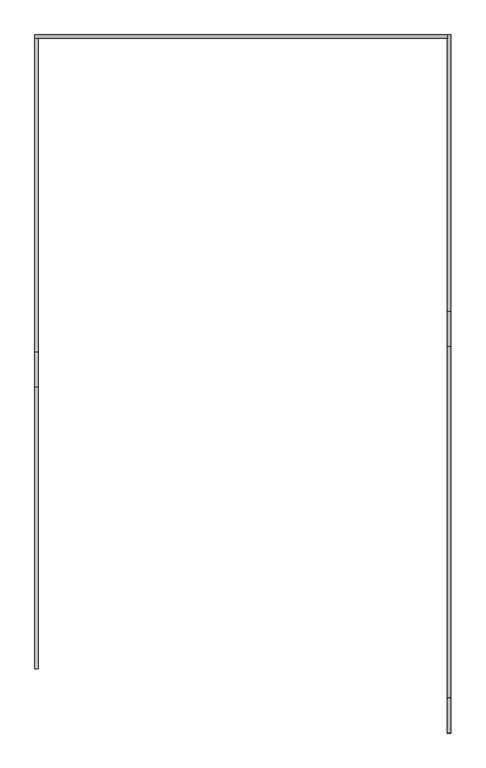
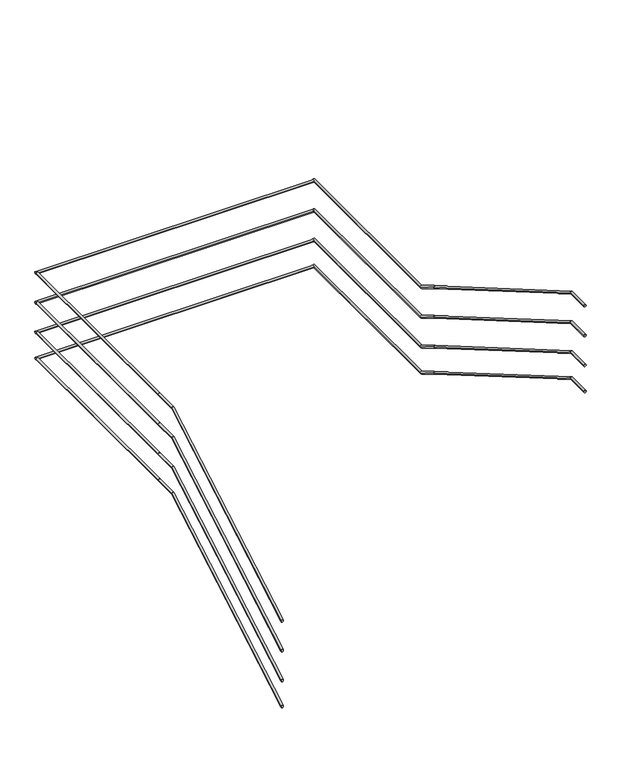
"""IFC4 building model written with IfcOpenShell, lengths in millimetres: railing geometry."""

import ifcopenshell
import ifcopenshell.guid

model = None  # the IFC model being written
_history = None  # IfcOwnerHistory: only IFC2X3 demands one
_inside = {}  # id of a spatial element -> (the spatial element, [elements in it])
_under = {}  # id of a project, library or spatial element -> (it, [spatial elements below it])
_declared = {}  # id of a project -> (the project, [libraries it declares])
_typed = {}  # id of a type object -> (the type object, [elements of that type])
_made_of = {}  # id of a material, layer set ... -> (it, [elements and type objects made of it])


def new_model(schema):
    """Start an empty IFC model of exactly this schema.

    Asked for "IFC4X3", IfcOpenShell would pick the latest addendum, in which some entities
    have other attributes; the version numbers below select the first issue.
    IFC2X3 requires an IfcOwnerHistory on every rooted entity: one is made here for all.
    """
    global model, _history
    if schema == "IFC4X3":
        model = ifcopenshell.file(schema_version=(4, 3, 0, 0))
    else:
        model = ifcopenshell.file(schema=schema)
    _inside.clear()
    _under.clear()
    _declared.clear()
    _typed.clear()
    _made_of.clear()
    _history = None
    if model.schema == "IFC2X3":
        org = make("IfcOrganization", Name="unknown")
        user = make(
            "IfcPersonAndOrganization",
            ThePerson=make("IfcPerson", FamilyName="unknown"),
            TheOrganization=org,
        )
        app = make(
            "IfcApplication",
            ApplicationDeveloper=org,
            Version="unknown",
            ApplicationFullName="unknown",
            ApplicationIdentifier="unknown",
        )
        _history = make(
            "IfcOwnerHistory",
            OwningUser=user,
            OwningApplication=app,
            ChangeAction="ADDED",
            CreationDate=0,
        )
    return model


def make(cls, **values):
    """One entity of the class cls with the attributes given. An attribute that is None is left unset."""
    return model.create_entity(
        cls, **{name: value for name, value in values.items() if value is not None}
    )


def rooted(cls, **values):
    """An entity with a GlobalId (a new one), such as an element, a storey or a relation."""
    return make(cls, GlobalId=ifcopenshell.guid.new(), OwnerHistory=_history, **values)


def si_unit(unit_type, name, prefix=None):
    """IfcSIUnit, for example si_unit("LENGTHUNIT", "METRE", prefix="MILLI")."""
    return make("IfcSIUnit", UnitType=unit_type, Prefix=prefix, Name=name)


def assignment(units):
    """IfcUnitAssignment: the units of a project."""
    return None if units is None else make("IfcUnitAssignment", Units=units)


def point(xyz):
    """IfcCartesianPoint."""
    return None if xyz is None else make("IfcCartesianPoint", Coordinates=xyz)


def direction(xyz):
    """IfcDirection."""
    return None if xyz is None else make("IfcDirection", DirectionRatios=xyz)


def frame(location, z_axis=None, x_axis=None):
    """IfcAxis2Placement3D, a coordinate frame: its origin and axes. An axis left out is left unset."""
    return make(
        "IfcAxis2Placement3D",
        Location=point(location),
        Axis=direction(z_axis),
        RefDirection=direction(x_axis),
    )


def origin():
    """The frame at (0, 0, 0) with its axes left unset."""
    return frame((0.0, 0.0, 0.0))


def place(relative_to, where):
    """IfcLocalPlacement: puts the frame where relative to a parent placement (None: the world)."""
    return make(
        "IfcLocalPlacement", PlacementRelTo=relative_to, RelativePlacement=where
    )


def context(
    kind, dimensions, precision=None, world=None, true_north=None, identifier=None
):
    """IfcGeometricRepresentationContext, for example the 3D "Model" context."""
    return make(
        "IfcGeometricRepresentationContext",
        ContextIdentifier=identifier,
        ContextType=kind,
        CoordinateSpaceDimension=dimensions,
        Precision=precision,
        WorldCoordinateSystem=world,
        TrueNorth=true_north,
    )


def project(units=None, contexts=None):
    """IfcProject with its units and contexts."""
    return rooted(
        "IfcProject",
        Name="project",
        RepresentationContexts=contexts,
        UnitsInContext=assignment(units),
    )


def spatial(cls, under=None, at=None, **own):
    """A site, building, storey or space (cls), placed at a placement, below another one or the project."""
    s = rooted(cls, ObjectPlacement=at, **own)
    if under is not None:
        _under.setdefault(under.id(), (under, []))[1].append(s)
    return s


def circle_curve(where, radius):
    """IfcCircle in the frame where."""
    return make("IfcCircle", Position=where, Radius=radius)


def ellipse_curve(where, semi_axis1, semi_axis2):
    """IfcEllipse in the frame where."""
    return make(
        "IfcEllipse", Position=where, SemiAxis1=semi_axis1, SemiAxis2=semi_axis2
    )


def shape(context_of_items, identifier, shape_type, items):
    """IfcShapeRepresentation: the items that make up one representation, for example the "Body"."""
    return make(
        "IfcShapeRepresentation",
        ContextOfItems=context_of_items,
        RepresentationIdentifier=identifier,
        RepresentationType=shape_type,
        Items=items,
    )


def source(mapping_origin, context_of_items, identifier, shape_type, items):
    """IfcRepresentationMap: a shape defined once, which mapped items show again and again."""
    return make(
        "IfcRepresentationMap",
        MappingOrigin=mapping_origin,
        MappedRepresentation=shape(context_of_items, identifier, shape_type, items),
    )


def transform(
    local_origin,
    x_axis=None,
    y_axis=None,
    z_axis=None,
    scale=None,
    scale2=None,
    scale3=None,
    uniform=True,
):
    """IfcCartesianTransformationOperator3D, or its non-uniform kind. x_axis, y_axis, z_axis: its Axis1, 2, 3."""
    if uniform:
        return make(
            "IfcCartesianTransformationOperator3D",
            Axis1=direction(x_axis),
            Axis2=direction(y_axis),
            LocalOrigin=point(local_origin),
            Scale=scale,
            Axis3=direction(z_axis),
        )
    return make(
        "IfcCartesianTransformationOperator3DnonUniform",
        Axis1=direction(x_axis),
        Axis2=direction(y_axis),
        LocalOrigin=point(local_origin),
        Scale=scale,
        Axis3=direction(z_axis),
        Scale2=scale2,
        Scale3=scale3,
    )


def mapped(mapping_source, mapping_target):
    """IfcMappedItem: shows the shape of a source again, moved by a transform."""
    return make(
        "IfcMappedItem", MappingSource=mapping_source, MappingTarget=mapping_target
    )


def made_of(thing, what):
    """Note that an element or type object is made of a material, layer set ...; save() writes the relation."""
    if what is not None:
        _made_of.setdefault(what.id(), (what, []))[1].append(thing)
    return thing


def element(
    cls,
    number,
    at=None,
    inside=None,
    cuts=None,
    type_object=None,
    material=None,
    context=None,
    identifier="Body",
    shape_type=None,
    held_by="IfcProductDefinitionShape",
    body=None,
    shapes=None,
    **own,
):
    """One element of the class cls, such as IfcWall. Its Tag is "e" and its number.

    at: its placement. inside: the storey or other place that contains it. cuts: it is an
    opening in that element (IfcRelVoidsElement). A single representation is given by context,
    identifier, shape_type and body (its items); several are given by shapes. held_by: the class
    of the entity that holds the representations. save() writes the other relations.
    """
    e = rooted(cls, Tag="e%d" % number, ObjectPlacement=at, **own)
    if body is not None:
        shapes = [shape(context, identifier, shape_type, body)]
    if shapes is not None:
        e.Representation = make(held_by, Representations=shapes)
    if inside is not None:
        _inside.setdefault(inside.id(), (inside, []))[1].append(e)
    if cuts is not None:
        rooted(
            "IfcRelVoidsElement", RelatingBuildingElement=cuts, RelatedOpeningElement=e
        )
    if type_object is not None:
        _typed.setdefault(type_object.id(), (type_object, []))[1].append(e)
    return made_of(e, material)


def aggregate(whole, parts):
    """IfcRelAggregates: a whole, such as a stair, and the parts it consists of."""
    return rooted("IfcRelAggregates", RelatingObject=whole, RelatedObjects=parts)


def save(model, path):
    """Write the relations noted so far, then the file.

    IfcRelAggregates (storeys below a building ...), IfcRelContainedInSpatialStructure (elements
    in a storey), IfcRelDefinesByType, IfcRelAssociatesMaterial and IfcRelDeclares: one each for
    every whole, place, type object, material and project.
    """
    for whole, parts in _under.values():
        aggregate(whole, parts)
    for where, things in _inside.values():
        rooted(
            "IfcRelContainedInSpatialStructure",
            RelatedElements=things,
            RelatingStructure=where,
        )
    for kind, things in _typed.values():
        rooted("IfcRelDefinesByType", RelatedObjects=things, RelatingType=kind)
    for what, things in _made_of.values():
        rooted("IfcRelAssociatesMaterial", RelatedObjects=things, RelatingMaterial=what)
    for by, libraries in _declared.values():
        rooted("IfcRelDeclares", RelatingContext=by, RelatedDefinitions=libraries)
    model.write(path)


def plane_surface(at):
    """IfcPlane: the flat surface through the origin of the frame at, square to its z axis."""
    return make("IfcPlane", Position=at)


def cylinder_surface(at, radius):
    """IfcCylindricalSurface: all points at the distance radius from the z axis of the frame at."""
    return make("IfcCylindricalSurface", Position=at, Radius=radius)


def advanced_brep(points, edges, surfaces, faces):
    """IfcAdvancedBrep: a solid bounded by faces that lie on surfaces and meet in shared edges.

    An edge is (start, end): straight between two places in points (the first is 0);
    or (start, end, curve); or (start, end, curve, False) where it runs against its curve.
    A face is (place in surfaces, loops), or (place, loops, False) where it looks against
    its surface's normal. A loop lists edges by number (the first is 1), with a minus sign
    where the edge is run from its end to its start. The first loop is the outer one.
    """
    corners = [point(p) for p in points]
    vertices = [make("IfcVertexPoint", VertexGeometry=c) for c in corners]
    made = []
    for start, end, *more in edges:
        made.append(
            make(
                "IfcEdgeCurve",
                EdgeStart=vertices[start],
                EdgeEnd=vertices[end],
                EdgeGeometry=more[0] if more else make("IfcPolyline", Points=[corners[start], corners[end]]),
                SameSense=more[1] if len(more) > 1 else True,
            )
        )
    hull = []
    for where, loops, *sense in faces:
        bounds = []
        for j, loop in enumerate(loops):
            ring = [make("IfcOrientedEdge", EdgeElement=made[abs(k) - 1], Orientation=k > 0) for k in loop]
            bounds.append(
                make(
                    "IfcFaceOuterBound" if j == 0 else "IfcFaceBound",
                    Bound=make("IfcEdgeLoop", EdgeList=ring),
                    Orientation=True,
                )
            )
        hull.append(make("IfcAdvancedFace", Bounds=bounds, FaceSurface=surfaces[where], SameSense=sense[0] if sense else True))
    return make("IfcAdvancedBrep", Outer=make("IfcClosedShell", CfsFaces=hull))


def railing_c3b53c4a(model_context):
    return source(origin(), model_context, "Body", "AdvancedBrep", [
        advanced_brep(
        [(51115.4, 12129.5208589, 7307.5963084), (51085.4, 12129.5208589, 7307.5963084), (51115.4, 14533.576096, 8709.9618634), (51085.4, 14533.576096, 8709.9618634), (51115.4, 14829.5208589, 8709.9618634), (51085.4, 14829.5208589, 8709.9618634)],
        [
            (0, 1, ellipse_curve(frame((51100.4, 12129.5208589, 7307.5963084), z_axis=(0.0, -1.0, 0.0), x_axis=(0.0, 0.0, -1.0)), 17.365555, 15.0)),
            (1, 0, ellipse_curve(frame((51100.4, 12129.5208589, 7307.5963084), z_axis=(0.0, -1.0, 0.0), x_axis=(0.0, 0.0, -1.0)), 17.365555, 15.0)),
            (0, 2),
            (2, 3, ellipse_curve(frame((51100.4, 14533.576096, 8709.9618634), z_axis=(0.0, -0.9653442134540491, -0.26097997921446625), x_axis=(0.0, 0.2609799792144657, -0.9653442134540494)), 15.5384989, 15.0)),
            (3, 1),
            (3, 2, ellipse_curve(frame((51100.4, 14533.576096, 8709.9618634), z_axis=(0.0, -0.9653442134540491, -0.26097997921446625), x_axis=(0.0, 0.2609799792144657, -0.9653442134540494)), 15.5384989, 15.0)),
            (4, 5, circle_curve(frame((51100.4, 14829.5208589, 8709.9618634), z_axis=(0.0, 1.0, 0.0), x_axis=(-1.0, 0.0, 0.0)), 15.0)),
            (5, 4, circle_curve(frame((51100.4, 14829.5208589, 8709.9618634), z_axis=(0.0, 1.0, 0.0), x_axis=(-1.0, 0.0, 0.0)), 15.0)),
            (2, 4),
            (5, 3),
        ],
        [
            plane_surface(frame((51100.4, 12129.5208589, 7324.9618634), z_axis=(0.0, -1.0, 0.0), x_axis=(0.0, 0.0, 1.0))),
            cylinder_surface(frame((51100.4, 12137.0789243, 7312.0051799), z_axis=(0.0, -0.8637789008984336, -0.5038710255240861), x_axis=(-1.0, 0.0, 0.0)), 15.0),
            plane_surface(frame((51100.4, 14829.5208589, 8724.9618634), z_axis=(0.0, 1.0, 0.0), x_axis=(0.0, 0.0, 1.0))),
            cylinder_surface(frame((51100.4, 14529.5208589, 8709.9618634), z_axis=(0.0, -1.0, 0.0), x_axis=(-1.0, 0.0, 0.0)), 15.0),
        ],
        [
            (0, [[1, 2]]),
            (1, [[-1, 3, 4, 5]]),
            (1, [[-2, -5, 6, -3]]),
            (2, [[7, 8]]),
            (3, [[-4, 9, -8, 10]]),
            (3, [[-6, -10, -7, -9]]),
        ],
    ),
        advanced_brep(
        [(51115.4, 14829.5208589, 8709.9618634), (51085.4, 14829.5208589, 8709.9618634), (51115.4, 17509.1208589, 8709.9618634), (51085.4, 17509.1208589, 8709.9618634)],
        [
            (0, 1, circle_curve(frame((51100.4, 14829.5208589, 8709.9618634), z_axis=(0.0, -1.0, 0.0), x_axis=(-1.0, 0.0, 0.0)), 15.0)),
            (1, 0, circle_curve(frame((51100.4, 14829.5208589, 8709.9618634), z_axis=(0.0, -1.0, 0.0), x_axis=(-1.0, 0.0, 0.0)), 15.0)),
            (2, 3, circle_curve(frame((51100.4, 17509.1208589, 8709.9618634), z_axis=(0.0, 1.0, 0.0), x_axis=(-1.0, 0.0, 0.0)), 15.0)),
            (3, 2, circle_curve(frame((51100.4, 17509.1208589, 8709.9618634), z_axis=(0.0, 1.0, 0.0), x_axis=(-1.0, 0.0, 0.0)), 15.0)),
            (0, 2),
            (3, 1),
        ],
        [
            plane_surface(frame((51100.4, 14829.5208589, 8724.9618634), z_axis=(0.0, -1.0, 0.0), x_axis=(0.0, 0.0, 1.0))),
            plane_surface(frame((51100.4, 17509.1208589, 8724.9618634), z_axis=(0.0, 1.0, 0.0), x_axis=(0.0, 0.0, 1.0))),
            cylinder_surface(frame((51100.4, 14829.5208589, 8709.9618634), z_axis=(0.0, -1.0, 0.0), x_axis=(-1.0, 0.0, 0.0)), 15.0),
        ],
        [
            (0, [[1, 2]]),
            (1, [[3, 4]]),
            (2, [[-1, 5, -4, 6]]),
            (2, [[-2, -6, -3, -5]]),
        ],
    ),
        advanced_brep(
        [(51085.4, 17509.1208589, 8709.9618634), (51085.4, 17539.1208589, 8709.9618634), (54609.6, 17509.1208589, 8709.9618634), (54609.6, 17539.1208589, 8709.9618634)],
        [
            (0, 1, circle_curve(frame((51085.4, 17524.1208589, 8709.9618634), z_axis=(-1.0, 0.0, 0.0), x_axis=(0.0, 1.0, 0.0)), 15.0)),
            (1, 0, circle_curve(frame((51085.4, 17524.1208589, 8709.9618634), z_axis=(-1.0, 0.0, 0.0), x_axis=(0.0, 1.0, 0.0)), 15.0)),
            (2, 3, circle_curve(frame((54609.6, 17524.1208589, 8709.9618634), z_axis=(1.0, 0.0, 0.0), x_axis=(0.0, 1.0, 0.0)), 15.0)),
            (3, 2, circle_curve(frame((54609.6, 17524.1208589, 8709.9618634), z_axis=(1.0, 0.0, 0.0), x_axis=(0.0, 1.0, 0.0)), 15.0)),
            (0, 2),
            (3, 1),
        ],
        [
            plane_surface(frame((51085.4, 17524.1208589, 8724.9618634), z_axis=(-1.0, 0.0, 0.0), x_axis=(0.0, 1.0, 0.0))),
            plane_surface(frame((54609.6, 17524.1208589, 8724.9618634), z_axis=(1.0, 0.0, 0.0), x_axis=(0.0, 1.0, 0.0))),
            cylinder_surface(frame((51085.4, 17524.1208589, 8709.9618634), z_axis=(-1.0, 0.0, 0.0), x_axis=(0.0, 1.0, 0.0)), 15.0),
        ],
        [
            (0, [[1, 2]]),
            (1, [[3, 4]]),
            (2, [[-1, 5, -4, 6]]),
            (2, [[-2, -6, -3, -5]]),
        ],
    ),
        advanced_brep(
        [(54609.6, 17539.1208589, 8709.9618634), (54639.6, 17539.1208589, 8709.9618634), (54609.6, 15175.4656218, 8709.9618634), (54639.6, 15175.4656218, 8709.9618634), (54609.6, 14879.5208589, 8882.5963084), (54639.6, 14879.5208589, 8882.5963084)],
        [
            (0, 1, circle_curve(frame((54624.6, 17539.1208589, 8709.9618634), z_axis=(0.0, 1.0, 0.0), x_axis=(1.0, 0.0, 0.0)), 15.0)),
            (1, 0, circle_curve(frame((54624.6, 17539.1208589, 8709.9618634), z_axis=(0.0, 1.0, 0.0), x_axis=(1.0, 0.0, 0.0)), 15.0)),
            (0, 2),
            (2, 3, ellipse_curve(frame((54624.6, 15175.4656218, 8709.9618634), z_axis=(0.0, 0.9653442134540493, -0.26097997921446586), x_axis=(0.0, 0.2609799792144653, 0.9653442134540493)), 15.5384989, 15.0)),
            (3, 1),
            (3, 2, ellipse_curve(frame((54624.6, 15175.4656218, 8709.9618634), z_axis=(0.0, 0.9653442134540493, -0.26097997921446586), x_axis=(0.0, 0.2609799792144653, 0.9653442134540493)), 15.5384989, 15.0)),
            (4, 5, ellipse_curve(frame((54624.6, 14879.5208589, 8882.5963084), z_axis=(0.0, -1.0, 0.0), x_axis=(0.0, 0.0, -1.0)), 17.365555, 15.0)),
            (5, 4, ellipse_curve(frame((54624.6, 14879.5208589, 8882.5963084), z_axis=(0.0, -1.0, 0.0), x_axis=(0.0, 0.0, -1.0)), 17.365555, 15.0)),
            (2, 4),
            (5, 3),
        ],
        [
            plane_surface(frame((54624.6, 17539.1208589, 8724.9618634), z_axis=(0.0, 1.0, 0.0), x_axis=(0.0, 0.0, -1.0))),
            cylinder_surface(frame((54624.6, 17539.1208589, 8709.9618634), z_axis=(0.0, 1.0, 0.0), x_axis=(1.0, 0.0, 0.0)), 15.0),
            plane_surface(frame((54624.6, 14879.5208589, 8899.9618634), z_axis=(0.0, -1.0, 0.0), x_axis=(0.0, 0.0, -1.0))),
            cylinder_surface(frame((54624.6, 15171.9627935, 8712.0051799), z_axis=(0.0, 0.8637789008984339, -0.5038710255240854), x_axis=(1.0, 0.0, 0.0)), 15.0),
        ],
        [
            (0, [[1, 2]]),
            (1, [[-1, 3, 4, 5]]),
            (1, [[-2, -5, 6, -3]]),
            (2, [[7, 8]]),
            (3, [[-4, 9, -8, 10]]),
            (3, [[-6, -10, -7, -9]]),
        ],
    ),
        advanced_brep(
        [(54609.6, 14879.5208589, 8882.5963084), (54639.6, 14879.5208589, 8882.5963084), (54609.6, 11875.4656218, 10634.9618634), (54639.6, 11875.4656218, 10634.9618634), (54609.6, 11579.5208589, 10634.9618634), (54639.6, 11579.5208589, 10634.9618634)],
        [
            (0, 1, ellipse_curve(frame((54624.6, 14879.5208589, 8882.5963084), z_axis=(0.0, 1.0, 0.0), x_axis=(0.0, 0.0, -1.0)), 17.365555, 15.0)),
            (1, 0, ellipse_curve(frame((54624.6, 14879.5208589, 8882.5963084), z_axis=(0.0, 1.0, 0.0), x_axis=(0.0, 0.0, -1.0)), 17.365555, 15.0)),
            (0, 2),
            (2, 3, ellipse_curve(frame((54624.6, 11875.4656218, 10634.9618634), z_axis=(0.0, 0.9653442134540491, -0.26097997921446625), x_axis=(0.0, -0.2609799792144661, -0.9653442134540492)), 15.5384989, 15.0)),
            (3, 1),
            (3, 2, ellipse_curve(frame((54624.6, 11875.4656218, 10634.9618634), z_axis=(0.0, 0.9653442134540491, -0.26097997921446625), x_axis=(0.0, -0.2609799792144661, -0.9653442134540492)), 15.5384989, 15.0)),
            (4, 5, circle_curve(frame((54624.6, 11579.5208589, 10634.9618634), z_axis=(0.0, -1.0, 0.0), x_axis=(1.0, 0.0, 0.0)), 15.0)),
            (5, 4, circle_curve(frame((54624.6, 11579.5208589, 10634.9618634), z_axis=(0.0, -1.0, 0.0), x_axis=(1.0, 0.0, 0.0)), 15.0)),
            (2, 4),
            (5, 3),
        ],
        [
            plane_surface(frame((54624.6, 14879.5208589, 8899.9618634), z_axis=(0.0, 1.0, 0.0), x_axis=(0.0, 0.0, -1.0))),
            cylinder_surface(frame((54624.6, 14871.9627935, 8887.0051799), z_axis=(0.0, 0.8637789008984335, -0.5038710255240861), x_axis=(1.0, 0.0, 0.0)), 15.0),
            plane_surface(frame((54624.6, 11579.5208589, 10649.9618634), z_axis=(0.0, -1.0, 0.0), x_axis=(0.0, 0.0, -1.0))),
            cylinder_surface(frame((54624.6, 11879.5208589, 10634.9618634), z_axis=(0.0, 1.0, 0.0), x_axis=(1.0, 0.0, 0.0)), 15.0),
        ],
        [
            (0, [[1, 2]]),
            (1, [[-1, 3, 4, 5]]),
            (1, [[-2, -5, 6, -3]]),
            (2, [[7, 8]]),
            (3, [[-4, 9, -8, 10]]),
            (3, [[-6, -10, -7, -9]]),
        ],
    ),
        advanced_brep(
        [(51115.4, 12129.5208589, 6507.5963084), (51085.4, 12129.5208589, 6507.5963084), (51115.4, 14533.576096, 7909.9618634), (51085.4, 14533.576096, 7909.9618634), (51115.4, 14829.5208589, 7909.9618634), (51085.4, 14829.5208589, 7909.9618634)],
        [
            (0, 1, ellipse_curve(frame((51100.4, 12129.5208589, 6507.5963084), z_axis=(0.0, -1.0, 0.0), x_axis=(0.0, 0.0, -1.0)), 17.365555, 15.0)),
            (1, 0, ellipse_curve(frame((51100.4, 12129.5208589, 6507.5963084), z_axis=(0.0, -1.0, 0.0), x_axis=(0.0, 0.0, -1.0)), 17.365555, 15.0)),
            (0, 2),
            (2, 3, ellipse_curve(frame((51100.4, 14533.576096, 7909.9618634), z_axis=(0.0, -0.9653442134540491, -0.26097997921446625), x_axis=(0.0, 0.2609799792144657, -0.9653442134540494)), 15.5384989, 15.0)),
            (3, 1),
            (3, 2, ellipse_curve(frame((51100.4, 14533.576096, 7909.9618634), z_axis=(0.0, -0.9653442134540491, -0.26097997921446625), x_axis=(0.0, 0.2609799792144657, -0.9653442134540494)), 15.5384989, 15.0)),
            (4, 5, circle_curve(frame((51100.4, 14829.5208589, 7909.9618634), z_axis=(0.0, 1.0, 0.0), x_axis=(-1.0, 0.0, 0.0)), 15.0)),
            (5, 4, circle_curve(frame((51100.4, 14829.5208589, 7909.9618634), z_axis=(0.0, 1.0, 0.0), x_axis=(-1.0, 0.0, 0.0)), 15.0)),
            (2, 4),
            (5, 3),
        ],
        [
            plane_surface(frame((51100.4, 12129.5208589, 6524.9618634), z_axis=(0.0, -1.0, 0.0), x_axis=(0.0, 0.0, 1.0))),
            cylinder_surface(frame((51100.4, 12137.0789243, 6512.0051799), z_axis=(0.0, -0.8637789008984336, -0.5038710255240861), x_axis=(-1.0, 0.0, 0.0)), 15.0),
            plane_surface(frame((51100.4, 14829.5208589, 7924.9618634), z_axis=(0.0, 1.0, 0.0), x_axis=(0.0, 0.0, 1.0))),
            cylinder_surface(frame((51100.4, 14529.5208589, 7909.9618634), z_axis=(0.0, -1.0, 0.0), x_axis=(-1.0, 0.0, 0.0)), 15.0),
        ],
        [
            (0, [[1, 2]]),
            (1, [[-1, 3, 4, 5]]),
            (1, [[-2, -5, 6, -3]]),
            (2, [[7, 8]]),
            (3, [[-4, 9, -8, 10]]),
            (3, [[-6, -10, -7, -9]]),
        ],
    ),
        advanced_brep(
        [(51115.4, 14829.5208589, 7909.9618634), (51085.4, 14829.5208589, 7909.9618634), (51115.4, 17509.1208589, 7909.9618634), (51085.4, 17509.1208589, 7909.9618634)],
        [
            (0, 1, circle_curve(frame((51100.4, 14829.5208589, 7909.9618634), z_axis=(0.0, -1.0, 0.0), x_axis=(-1.0, 0.0, 0.0)), 15.0)),
            (1, 0, circle_curve(frame((51100.4, 14829.5208589, 7909.9618634), z_axis=(0.0, -1.0, 0.0), x_axis=(-1.0, 0.0, 0.0)), 15.0)),
            (2, 3, circle_curve(frame((51100.4, 17509.1208589, 7909.9618634), z_axis=(0.0, 1.0, 0.0), x_axis=(-1.0, 0.0, 0.0)), 15.0)),
            (3, 2, circle_curve(frame((51100.4, 17509.1208589, 7909.9618634), z_axis=(0.0, 1.0, 0.0), x_axis=(-1.0, 0.0, 0.0)), 15.0)),
            (0, 2),
            (3, 1),
        ],
        [
            plane_surface(frame((51100.4, 14829.5208589, 7924.9618634), z_axis=(0.0, -1.0, 0.0), x_axis=(0.0, 0.0, 1.0))),
            plane_surface(frame((51100.4, 17509.1208589, 7924.9618634), z_axis=(0.0, 1.0, 0.0), x_axis=(0.0, 0.0, 1.0))),
            cylinder_surface(frame((51100.4, 14829.5208589, 7909.9618634), z_axis=(0.0, -1.0, 0.0), x_axis=(-1.0, 0.0, 0.0)), 15.0),
        ],
        [
            (0, [[1, 2]]),
            (1, [[3, 4]]),
            (2, [[-1, 5, -4, 6]]),
            (2, [[-2, -6, -3, -5]]),
        ],
    ),
        advanced_brep(
        [(51085.4, 17509.1208589, 7909.9618634), (51085.4, 17539.1208589, 7909.9618634), (54609.6, 17509.1208589, 7909.9618634), (54609.6, 17539.1208589, 7909.9618634)],
        [
            (0, 1, circle_curve(frame((51085.4, 17524.1208589, 7909.9618634), z_axis=(-1.0, 0.0, 0.0), x_axis=(0.0, 1.0, 0.0)), 15.0)),
            (1, 0, circle_curve(frame((51085.4, 17524.1208589, 7909.9618634), z_axis=(-1.0, 0.0, 0.0), x_axis=(0.0, 1.0, 0.0)), 15.0)),
            (2, 3, circle_curve(frame((54609.6, 17524.1208589, 7909.9618634), z_axis=(1.0, 0.0, 0.0), x_axis=(0.0, 1.0, 0.0)), 15.0)),
            (3, 2, circle_curve(frame((54609.6, 17524.1208589, 7909.9618634), z_axis=(1.0, 0.0, 0.0), x_axis=(0.0, 1.0, 0.0)), 15.0)),
            (0, 2),
            (3, 1),
        ],
        [
            plane_surface(frame((51085.4, 17524.1208589, 7924.9618634), z_axis=(-1.0, 0.0, 0.0), x_axis=(0.0, 1.0, 0.0))),
            plane_surface(frame((54609.6, 17524.1208589, 7924.9618634), z_axis=(1.0, 0.0, 0.0), x_axis=(0.0, 1.0, 0.0))),
            cylinder_surface(frame((51085.4, 17524.1208589, 7909.9618634), z_axis=(-1.0, 0.0, 0.0), x_axis=(0.0, 1.0, 0.0)), 15.0),
        ],
        [
            (0, [[1, 2]]),
            (1, [[3, 4]]),
            (2, [[-1, 5, -4, 6]]),
            (2, [[-2, -6, -3, -5]]),
        ],
    ),
        advanced_brep(
        [(54609.6, 17539.1208589, 7909.9618634), (54639.6, 17539.1208589, 7909.9618634), (54609.6, 15175.4656218, 7909.9618634), (54639.6, 15175.4656218, 7909.9618634), (54609.6, 14879.5208589, 8082.5963084), (54639.6, 14879.5208589, 8082.5963084)],
        [
            (0, 1, circle_curve(frame((54624.6, 17539.1208589, 7909.9618634), z_axis=(0.0, 1.0, 0.0), x_axis=(1.0, 0.0, 0.0)), 15.0)),
            (1, 0, circle_curve(frame((54624.6, 17539.1208589, 7909.9618634), z_axis=(0.0, 1.0, 0.0), x_axis=(1.0, 0.0, 0.0)), 15.0)),
            (0, 2),
            (2, 3, ellipse_curve(frame((54624.6, 15175.4656218, 7909.9618634), z_axis=(0.0, 0.9653442134540493, -0.26097997921446586), x_axis=(0.0, 0.2609799792144653, 0.9653442134540493)), 15.5384989, 15.0)),
            (3, 1),
            (3, 2, ellipse_curve(frame((54624.6, 15175.4656218, 7909.9618634), z_axis=(0.0, 0.9653442134540493, -0.26097997921446586), x_axis=(0.0, 0.2609799792144653, 0.9653442134540493)), 15.5384989, 15.0)),
            (4, 5, ellipse_curve(frame((54624.6, 14879.5208589, 8082.5963084), z_axis=(0.0, -1.0, 0.0), x_axis=(0.0, 0.0, -1.0)), 17.365555, 15.0)),
            (5, 4, ellipse_curve(frame((54624.6, 14879.5208589, 8082.5963084), z_axis=(0.0, -1.0, 0.0), x_axis=(0.0, 0.0, -1.0)), 17.365555, 15.0)),
            (2, 4),
            (5, 3),
        ],
        [
            plane_surface(frame((54624.6, 17539.1208589, 7924.9618634), z_axis=(0.0, 1.0, 0.0), x_axis=(0.0, 0.0, -1.0))),
            cylinder_surface(frame((54624.6, 17539.1208589, 7909.9618634), z_axis=(0.0, 1.0, 0.0), x_axis=(1.0, 0.0, 0.0)), 15.0),
            plane_surface(frame((54624.6, 14879.5208589, 8099.9618634), z_axis=(0.0, -1.0, 0.0), x_axis=(0.0, 0.0, -1.0))),
            cylinder_surface(frame((54624.6, 15171.9627935, 7912.0051799), z_axis=(0.0, 0.8637789008984339, -0.5038710255240854), x_axis=(1.0, 0.0, 0.0)), 15.0),
        ],
        [
            (0, [[1, 2]]),
            (1, [[-1, 3, 4, 5]]),
            (1, [[-2, -5, 6, -3]]),
            (2, [[7, 8]]),
            (3, [[-4, 9, -8, 10]]),
            (3, [[-6, -10, -7, -9]]),
        ],
    ),
        advanced_brep(
        [(54609.6, 14879.5208589, 8082.5963084), (54639.6, 14879.5208589, 8082.5963084), (54609.6, 11875.4656218, 9834.9618634), (54639.6, 11875.4656218, 9834.9618634), (54609.6, 11579.5208589, 9834.9618634), (54639.6, 11579.5208589, 9834.9618634)],
        [
            (0, 1, ellipse_curve(frame((54624.6, 14879.5208589, 8082.5963084), z_axis=(0.0, 1.0, 0.0), x_axis=(0.0, 0.0, -1.0)), 17.365555, 15.0)),
            (1, 0, ellipse_curve(frame((54624.6, 14879.5208589, 8082.5963084), z_axis=(0.0, 1.0, 0.0), x_axis=(0.0, 0.0, -1.0)), 17.365555, 15.0)),
            (0, 2),
            (2, 3, ellipse_curve(frame((54624.6, 11875.4656218, 9834.9618634), z_axis=(0.0, 0.9653442134540491, -0.26097997921446625), x_axis=(0.0, -0.2609799792144661, -0.9653442134540492)), 15.5384989, 15.0)),
            (3, 1),
            (3, 2, ellipse_curve(frame((54624.6, 11875.4656218, 9834.9618634), z_axis=(0.0, 0.9653442134540491, -0.26097997921446625), x_axis=(0.0, -0.2609799792144661, -0.9653442134540492)), 15.5384989, 15.0)),
            (4, 5, circle_curve(frame((54624.6, 11579.5208589, 9834.9618634), z_axis=(0.0, -1.0, 0.0), x_axis=(1.0, 0.0, 0.0)), 15.0)),
            (5, 4, circle_curve(frame((54624.6, 11579.5208589, 9834.9618634), z_axis=(0.0, -1.0, 0.0), x_axis=(1.0, 0.0, 0.0)), 15.0)),
            (2, 4),
            (5, 3),
        ],
        [
            plane_surface(frame((54624.6, 14879.5208589, 8099.9618634), z_axis=(0.0, 1.0, 0.0), x_axis=(0.0, 0.0, -1.0))),
            cylinder_surface(frame((54624.6, 14871.9627935, 8087.0051799), z_axis=(0.0, 0.8637789008984335, -0.5038710255240861), x_axis=(1.0, 0.0, 0.0)), 15.0),
            plane_surface(frame((54624.6, 11579.5208589, 9849.9618634), z_axis=(0.0, -1.0, 0.0), x_axis=(0.0, 0.0, -1.0))),
            cylinder_surface(frame((54624.6, 11879.5208589, 9834.9618634), z_axis=(0.0, 1.0, 0.0), x_axis=(1.0, 0.0, 0.0)), 15.0),
        ],
        [
            (0, [[1, 2]]),
            (1, [[-1, 3, 4, 5]]),
            (1, [[-2, -5, 6, -3]]),
            (2, [[7, 8]]),
            (3, [[-4, 9, -8, 10]]),
            (3, [[-6, -10, -7, -9]]),
        ],
    ),
        advanced_brep(
        [(51115.4, 12129.5208589, 6907.5963084), (51085.4, 12129.5208589, 6907.5963084), (51115.4, 14533.576096, 8309.9618634), (51085.4, 14533.576096, 8309.9618634), (51115.4, 14829.5208589, 8309.9618634), (51085.4, 14829.5208589, 8309.9618634)],
        [
            (0, 1, ellipse_curve(frame((51100.4, 12129.5208589, 6907.5963084), z_axis=(0.0, -1.0, 0.0), x_axis=(0.0, 0.0, -1.0)), 17.365555, 15.0)),
            (1, 0, ellipse_curve(frame((51100.4, 12129.5208589, 6907.5963084), z_axis=(0.0, -1.0, 0.0), x_axis=(0.0, 0.0, -1.0)), 17.365555, 15.0)),
            (0, 2),
            (2, 3, ellipse_curve(frame((51100.4, 14533.576096, 8309.9618634), z_axis=(0.0, -0.9653442134540491, -0.26097997921446625), x_axis=(0.0, 0.2609799792144657, -0.9653442134540494)), 15.5384989, 15.0)),
            (3, 1),
            (3, 2, ellipse_curve(frame((51100.4, 14533.576096, 8309.9618634), z_axis=(0.0, -0.9653442134540491, -0.26097997921446625), x_axis=(0.0, 0.2609799792144657, -0.9653442134540494)), 15.5384989, 15.0)),
            (4, 5, circle_curve(frame((51100.4, 14829.5208589, 8309.9618634), z_axis=(0.0, 1.0, 0.0), x_axis=(-1.0, 0.0, 0.0)), 15.0)),
            (5, 4, circle_curve(frame((51100.4, 14829.5208589, 8309.9618634), z_axis=(0.0, 1.0, 0.0), x_axis=(-1.0, 0.0, 0.0)), 15.0)),
            (2, 4),
            (5, 3),
        ],
        [
            plane_surface(frame((51100.4, 12129.5208589, 6924.9618634), z_axis=(0.0, -1.0, 0.0), x_axis=(0.0, 0.0, 1.0))),
            cylinder_surface(frame((51100.4, 12137.0789243, 6912.0051799), z_axis=(0.0, -0.8637789008984336, -0.5038710255240861), x_axis=(-1.0, 0.0, 0.0)), 15.0),
            plane_surface(frame((51100.4, 14829.5208589, 8324.9618634), z_axis=(0.0, 1.0, 0.0), x_axis=(0.0, 0.0, 1.0))),
            cylinder_surface(frame((51100.4, 14529.5208589, 8309.9618634), z_axis=(0.0, -1.0, 0.0), x_axis=(-1.0, 0.0, 0.0)), 15.0),
        ],
        [
            (0, [[1, 2]]),
            (1, [[-1, 3, 4, 5]]),
            (1, [[-2, -5, 6, -3]]),
            (2, [[7, 8]]),
            (3, [[-4, 9, -8, 10]]),
            (3, [[-6, -10, -7, -9]]),
        ],
    ),
        advanced_brep(
        [(51115.4, 14829.5208589, 8309.9618634), (51085.4, 14829.5208589, 8309.9618634), (51115.4, 17509.1208589, 8309.9618634), (51085.4, 17509.1208589, 8309.9618634)],
        [
            (0, 1, circle_curve(frame((51100.4, 14829.5208589, 8309.9618634), z_axis=(0.0, -1.0, 0.0), x_axis=(-1.0, 0.0, 0.0)), 15.0)),
            (1, 0, circle_curve(frame((51100.4, 14829.5208589, 8309.9618634), z_axis=(0.0, -1.0, 0.0), x_axis=(-1.0, 0.0, 0.0)), 15.0)),
            (2, 3, circle_curve(frame((51100.4, 17509.1208589, 8309.9618634), z_axis=(0.0, 1.0, 0.0), x_axis=(-1.0, 0.0, 0.0)), 15.0)),
            (3, 2, circle_curve(frame((51100.4, 17509.1208589, 8309.9618634), z_axis=(0.0, 1.0, 0.0), x_axis=(-1.0, 0.0, 0.0)), 15.0)),
            (0, 2),
            (3, 1),
        ],
        [
            plane_surface(frame((51100.4, 14829.5208589, 8324.9618634), z_axis=(0.0, -1.0, 0.0), x_axis=(0.0, 0.0, 1.0))),
            plane_surface(frame((51100.4, 17509.1208589, 8324.9618634), z_axis=(0.0, 1.0, 0.0), x_axis=(0.0, 0.0, 1.0))),
            cylinder_surface(frame((51100.4, 14829.5208589, 8309.9618634), z_axis=(0.0, -1.0, 0.0), x_axis=(-1.0, 0.0, 0.0)), 15.0),
        ],
        [
            (0, [[1, 2]]),
            (1, [[3, 4]]),
            (2, [[-1, 5, -4, 6]]),
            (2, [[-2, -6, -3, -5]]),
        ],
    ),
        advanced_brep(
        [(51085.4, 17509.1208589, 8309.9618634), (51085.4, 17539.1208589, 8309.9618634), (54609.6, 17509.1208589, 8309.9618634), (54609.6, 17539.1208589, 8309.9618634)],
        [
            (0, 1, circle_curve(frame((51085.4, 17524.1208589, 8309.9618634), z_axis=(-1.0, 0.0, 0.0), x_axis=(0.0, 1.0, 0.0)), 15.0)),
            (1, 0, circle_curve(frame((51085.4, 17524.1208589, 8309.9618634), z_axis=(-1.0, 0.0, 0.0), x_axis=(0.0, 1.0, 0.0)), 15.0)),
            (2, 3, circle_curve(frame((54609.6, 17524.1208589, 8309.9618634), z_axis=(1.0, 0.0, 0.0), x_axis=(0.0, 1.0, 0.0)), 15.0)),
            (3, 2, circle_curve(frame((54609.6, 17524.1208589, 8309.9618634), z_axis=(1.0, 0.0, 0.0), x_axis=(0.0, 1.0, 0.0)), 15.0)),
            (0, 2),
            (3, 1),
        ],
        [
            plane_surface(frame((51085.4, 17524.1208589, 8324.9618634), z_axis=(-1.0, 0.0, 0.0), x_axis=(0.0, 1.0, 0.0))),
            plane_surface(frame((54609.6, 17524.1208589, 8324.9618634), z_axis=(1.0, 0.0, 0.0), x_axis=(0.0, 1.0, 0.0))),
            cylinder_surface(frame((51085.4, 17524.1208589, 8309.9618634), z_axis=(-1.0, 0.0, 0.0), x_axis=(0.0, 1.0, 0.0)), 15.0),
        ],
        [
            (0, [[1, 2]]),
            (1, [[3, 4]]),
            (2, [[-1, 5, -4, 6]]),
            (2, [[-2, -6, -3, -5]]),
        ],
    ),
        advanced_brep(
        [(54609.6, 17539.1208589, 8309.9618634), (54639.6, 17539.1208589, 8309.9618634), (54609.6, 15175.4656218, 8309.9618634), (54639.6, 15175.4656218, 8309.9618634), (54609.6, 14879.5208589, 8482.5963084), (54639.6, 14879.5208589, 8482.5963084)],
        [
            (0, 1, circle_curve(frame((54624.6, 17539.1208589, 8309.9618634), z_axis=(0.0, 1.0, 0.0), x_axis=(1.0, 0.0, 0.0)), 15.0)),
            (1, 0, circle_curve(frame((54624.6, 17539.1208589, 8309.9618634), z_axis=(0.0, 1.0, 0.0), x_axis=(1.0, 0.0, 0.0)), 15.0)),
            (0, 2),
            (2, 3, ellipse_curve(frame((54624.6, 15175.4656218, 8309.9618634), z_axis=(0.0, 0.9653442134540493, -0.26097997921446586), x_axis=(0.0, 0.2609799792144653, 0.9653442134540493)), 15.5384989, 15.0)),
            (3, 1),
            (3, 2, ellipse_curve(frame((54624.6, 15175.4656218, 8309.9618634), z_axis=(0.0, 0.9653442134540493, -0.26097997921446586), x_axis=(0.0, 0.2609799792144653, 0.9653442134540493)), 15.5384989, 15.0)),
            (4, 5, ellipse_curve(frame((54624.6, 14879.5208589, 8482.5963084), z_axis=(0.0, -1.0, 0.0), x_axis=(0.0, 0.0, -1.0)), 17.365555, 15.0)),
            (5, 4, ellipse_curve(frame((54624.6, 14879.5208589, 8482.5963084), z_axis=(0.0, -1.0, 0.0), x_axis=(0.0, 0.0, -1.0)), 17.365555, 15.0)),
            (2, 4),
            (5, 3),
        ],
        [
            plane_surface(frame((54624.6, 17539.1208589, 8324.9618634), z_axis=(0.0, 1.0, 0.0), x_axis=(0.0, 0.0, -1.0))),
            cylinder_surface(frame((54624.6, 17539.1208589, 8309.9618634), z_axis=(0.0, 1.0, 0.0), x_axis=(1.0, 0.0, 0.0)), 15.0),
            plane_surface(frame((54624.6, 14879.5208589, 8499.9618634), z_axis=(0.0, -1.0, 0.0), x_axis=(0.0, 0.0, -1.0))),
            cylinder_surface(frame((54624.6, 15171.9627935, 8312.0051799), z_axis=(0.0, 0.8637789008984339, -0.5038710255240854), x_axis=(1.0, 0.0, 0.0)), 15.0),
        ],
        [
            (0, [[1, 2]]),
            (1, [[-1, 3, 4, 5]]),
            (1, [[-2, -5, 6, -3]]),
            (2, [[7, 8]]),
            (3, [[-4, 9, -8, 10]]),
            (3, [[-6, -10, -7, -9]]),
        ],
    ),
        advanced_brep(
        [(54609.6, 14879.5208589, 8482.5963084), (54639.6, 14879.5208589, 8482.5963084), (54609.6, 11875.4656218, 10234.9618634), (54639.6, 11875.4656218, 10234.9618634), (54609.6, 11579.5208589, 10234.9618634), (54639.6, 11579.5208589, 10234.9618634)],
        [
            (0, 1, ellipse_curve(frame((54624.6, 14879.5208589, 8482.5963084), z_axis=(0.0, 1.0, 0.0), x_axis=(0.0, 0.0, -1.0)), 17.365555, 15.0)),
            (1, 0, ellipse_curve(frame((54624.6, 14879.5208589, 8482.5963084), z_axis=(0.0, 1.0, 0.0), x_axis=(0.0, 0.0, -1.0)), 17.365555, 15.0)),
            (0, 2),
            (2, 3, ellipse_curve(frame((54624.6, 11875.4656218, 10234.9618634), z_axis=(0.0, 0.9653442134540491, -0.26097997921446625), x_axis=(0.0, -0.2609799792144661, -0.9653442134540492)), 15.5384989, 15.0)),
            (3, 1),
            (3, 2, ellipse_curve(frame((54624.6, 11875.4656218, 10234.9618634), z_axis=(0.0, 0.9653442134540491, -0.26097997921446625), x_axis=(0.0, -0.2609799792144661, -0.9653442134540492)), 15.5384989, 15.0)),
            (4, 5, circle_curve(frame((54624.6, 11579.5208589, 10234.9618634), z_axis=(0.0, -1.0, 0.0), x_axis=(1.0, 0.0, 0.0)), 15.0)),
            (5, 4, circle_curve(frame((54624.6, 11579.5208589, 10234.9618634), z_axis=(0.0, -1.0, 0.0), x_axis=(1.0, 0.0, 0.0)), 15.0)),
            (2, 4),
            (5, 3),
        ],
        [
            plane_surface(frame((54624.6, 14879.5208589, 8499.9618634), z_axis=(0.0, 1.0, 0.0), x_axis=(0.0, 0.0, -1.0))),
            cylinder_surface(frame((54624.6, 14871.9627935, 8487.0051799), z_axis=(0.0, 0.8637789008984335, -0.5038710255240861), x_axis=(1.0, 0.0, 0.0)), 15.0),
            plane_surface(frame((54624.6, 11579.5208589, 10249.9618634), z_axis=(0.0, -1.0, 0.0), x_axis=(0.0, 0.0, -1.0))),
            cylinder_surface(frame((54624.6, 11879.5208589, 10234.9618634), z_axis=(0.0, 1.0, 0.0), x_axis=(1.0, 0.0, 0.0)), 15.0),
        ],
        [
            (0, [[1, 2]]),
            (1, [[-1, 3, 4, 5]]),
            (1, [[-2, -5, 6, -3]]),
            (2, [[7, 8]]),
            (3, [[-4, 9, -8, 10]]),
            (3, [[-6, -10, -7, -9]]),
        ],
    ),
        advanced_brep(
        [(51115.4, 12129.5208589, 6157.5963084), (51085.4, 12129.5208589, 6157.5963084), (51115.4, 14533.576096, 7559.9618634), (51085.4, 14533.576096, 7559.9618634), (51115.4, 14829.5208589, 7559.9618634), (51085.4, 14829.5208589, 7559.9618634)],
        [
            (0, 1, ellipse_curve(frame((51100.4, 12129.5208589, 6157.5963084), z_axis=(0.0, -1.0, 0.0), x_axis=(0.0, 0.0, -1.0)), 17.365555, 15.0)),
            (1, 0, ellipse_curve(frame((51100.4, 12129.5208589, 6157.5963084), z_axis=(0.0, -1.0, 0.0), x_axis=(0.0, 0.0, -1.0)), 17.365555, 15.0)),
            (0, 2),
            (2, 3, ellipse_curve(frame((51100.4, 14533.576096, 7559.9618634), z_axis=(0.0, -0.9653442134540491, -0.26097997921446625), x_axis=(0.0, 0.2609799792144657, -0.9653442134540494)), 15.5384989, 15.0)),
            (3, 1),
            (3, 2, ellipse_curve(frame((51100.4, 14533.576096, 7559.9618634), z_axis=(0.0, -0.9653442134540491, -0.26097997921446625), x_axis=(0.0, 0.2609799792144657, -0.9653442134540494)), 15.5384989, 15.0)),
            (4, 5, circle_curve(frame((51100.4, 14829.5208589, 7559.9618634), z_axis=(0.0, 1.0, 0.0), x_axis=(-1.0, 0.0, 0.0)), 15.0)),
            (5, 4, circle_curve(frame((51100.4, 14829.5208589, 7559.9618634), z_axis=(0.0, 1.0, 0.0), x_axis=(-1.0, 0.0, 0.0)), 15.0)),
            (2, 4),
            (5, 3),
        ],
        [
            plane_surface(frame((51100.4, 12129.5208589, 6174.9618634), z_axis=(0.0, -1.0, 0.0), x_axis=(0.0, 0.0, 1.0))),
            cylinder_surface(frame((51100.4, 12137.0789243, 6162.0051799), z_axis=(0.0, -0.8637789008984336, -0.5038710255240861), x_axis=(-1.0, 0.0, 0.0)), 15.0),
            plane_surface(frame((51100.4, 14829.5208589, 7574.9618634), z_axis=(0.0, 1.0, 0.0), x_axis=(0.0, 0.0, 1.0))),
            cylinder_surface(frame((51100.4, 14529.5208589, 7559.9618634), z_axis=(0.0, -1.0, 0.0), x_axis=(-1.0, 0.0, 0.0)), 15.0),
        ],
        [
            (0, [[1, 2]]),
            (1, [[-1, 3, 4, 5]]),
            (1, [[-2, -5, 6, -3]]),
            (2, [[7, 8]]),
            (3, [[-4, 9, -8, 10]]),
            (3, [[-6, -10, -7, -9]]),
        ],
    ),
        advanced_brep(
        [(51115.4, 14829.5208589, 7559.9618634), (51085.4, 14829.5208589, 7559.9618634), (51115.4, 17509.1208589, 7559.9618634), (51085.4, 17509.1208589, 7559.9618634)],
        [
            (0, 1, circle_curve(frame((51100.4, 14829.5208589, 7559.9618634), z_axis=(0.0, -1.0, 0.0), x_axis=(-1.0, 0.0, 0.0)), 15.0)),
            (1, 0, circle_curve(frame((51100.4, 14829.5208589, 7559.9618634), z_axis=(0.0, -1.0, 0.0), x_axis=(-1.0, 0.0, 0.0)), 15.0)),
            (2, 3, circle_curve(frame((51100.4, 17509.1208589, 7559.9618634), z_axis=(0.0, 1.0, 0.0), x_axis=(-1.0, 0.0, 0.0)), 15.0)),
            (3, 2, circle_curve(frame((51100.4, 17509.1208589, 7559.9618634), z_axis=(0.0, 1.0, 0.0), x_axis=(-1.0, 0.0, 0.0)), 15.0)),
            (0, 2),
            (3, 1),
        ],
        [
            plane_surface(frame((51100.4, 14829.5208589, 7574.9618634), z_axis=(0.0, -1.0, 0.0), x_axis=(0.0, 0.0, 1.0))),
            plane_surface(frame((51100.4, 17509.1208589, 7574.9618634), z_axis=(0.0, 1.0, 0.0), x_axis=(0.0, 0.0, 1.0))),
            cylinder_surface(frame((51100.4, 14829.5208589, 7559.9618634), z_axis=(0.0, -1.0, 0.0), x_axis=(-1.0, 0.0, 0.0)), 15.0),
        ],
        [
            (0, [[1, 2]]),
            (1, [[3, 4]]),
            (2, [[-1, 5, -4, 6]]),
            (2, [[-2, -6, -3, -5]]),
        ],
    ),
        advanced_brep(
        [(51085.4, 17509.1208589, 7559.9618634), (51085.4, 17539.1208589, 7559.9618634), (54609.6, 17509.1208589, 7559.9618634), (54609.6, 17539.1208589, 7559.9618634)],
        [
            (0, 1, circle_curve(frame((51085.4, 17524.1208589, 7559.9618634), z_axis=(-1.0, 0.0, 0.0), x_axis=(0.0, 1.0, 0.0)), 15.0)),
            (1, 0, circle_curve(frame((51085.4, 17524.1208589, 7559.9618634), z_axis=(-1.0, 0.0, 0.0), x_axis=(0.0, 1.0, 0.0)), 15.0)),
            (2, 3, circle_curve(frame((54609.6, 17524.1208589, 7559.9618634), z_axis=(1.0, 0.0, 0.0), x_axis=(0.0, 1.0, 0.0)), 15.0)),
            (3, 2, circle_curve(frame((54609.6, 17524.1208589, 7559.9618634), z_axis=(1.0, 0.0, 0.0), x_axis=(0.0, 1.0, 0.0)), 15.0)),
            (0, 2),
            (3, 1),
        ],
        [
            plane_surface(frame((51085.4, 17524.1208589, 7574.9618634), z_axis=(-1.0, 0.0, 0.0), x_axis=(0.0, 1.0, 0.0))),
            plane_surface(frame((54609.6, 17524.1208589, 7574.9618634), z_axis=(1.0, 0.0, 0.0), x_axis=(0.0, 1.0, 0.0))),
            cylinder_surface(frame((51085.4, 17524.1208589, 7559.9618634), z_axis=(-1.0, 0.0, 0.0), x_axis=(0.0, 1.0, 0.0)), 15.0),
        ],
        [
            (0, [[1, 2]]),
            (1, [[3, 4]]),
            (2, [[-1, 5, -4, 6]]),
            (2, [[-2, -6, -3, -5]]),
        ],
    ),
        advanced_brep(
        [(54609.6, 17539.1208589, 7559.9618634), (54639.6, 17539.1208589, 7559.9618634), (54609.6, 15175.4656218, 7559.9618634), (54639.6, 15175.4656218, 7559.9618634), (54609.6, 14879.5208589, 7732.5963084), (54639.6, 14879.5208589, 7732.5963084)],
        [
            (0, 1, circle_curve(frame((54624.6, 17539.1208589, 7559.9618634), z_axis=(0.0, 1.0, 0.0), x_axis=(1.0, 0.0, 0.0)), 15.0)),
            (1, 0, circle_curve(frame((54624.6, 17539.1208589, 7559.9618634), z_axis=(0.0, 1.0, 0.0), x_axis=(1.0, 0.0, 0.0)), 15.0)),
            (0, 2),
            (2, 3, ellipse_curve(frame((54624.6, 15175.4656218, 7559.9618634), z_axis=(0.0, 0.9653442134540493, -0.26097997921446586), x_axis=(0.0, 0.2609799792144653, 0.9653442134540493)), 15.5384989, 15.0)),
            (3, 1),
            (3, 2, ellipse_curve(frame((54624.6, 15175.4656218, 7559.9618634), z_axis=(0.0, 0.9653442134540493, -0.26097997921446586), x_axis=(0.0, 0.2609799792144653, 0.9653442134540493)), 15.5384989, 15.0)),
            (4, 5, ellipse_curve(frame((54624.6, 14879.5208589, 7732.5963084), z_axis=(0.0, -1.0, 0.0), x_axis=(0.0, 0.0, -1.0)), 17.365555, 15.0)),
            (5, 4, ellipse_curve(frame((54624.6, 14879.5208589, 7732.5963084), z_axis=(0.0, -1.0, 0.0), x_axis=(0.0, 0.0, -1.0)), 17.365555, 15.0)),
            (2, 4),
            (5, 3),
        ],
        [
            plane_surface(frame((54624.6, 17539.1208589, 7574.9618634), z_axis=(0.0, 1.0, 0.0), x_axis=(0.0, 0.0, -1.0))),
            cylinder_surface(frame((54624.6, 17539.1208589, 7559.9618634), z_axis=(0.0, 1.0, 0.0), x_axis=(1.0, 0.0, 0.0)), 15.0),
            plane_surface(frame((54624.6, 14879.5208589, 7749.9618634), z_axis=(0.0, -1.0, 0.0), x_axis=(0.0, 0.0, -1.0))),
            cylinder_surface(frame((54624.6, 15171.9627935, 7562.0051799), z_axis=(0.0, 0.8637789008984339, -0.5038710255240854), x_axis=(1.0, 0.0, 0.0)), 15.0),
        ],
        [
            (0, [[1, 2]]),
            (1, [[-1, 3, 4, 5]]),
            (1, [[-2, -5, 6, -3]]),
            (2, [[7, 8]]),
            (3, [[-4, 9, -8, 10]]),
            (3, [[-6, -10, -7, -9]]),
        ],
    ),
        advanced_brep(
        [(54609.6, 14879.5208589, 7732.5963084), (54639.6, 14879.5208589, 7732.5963084), (54609.6, 11875.4656218, 9484.9618634), (54639.6, 11875.4656218, 9484.9618634), (54609.6, 11579.5208589, 9484.9618634), (54639.6, 11579.5208589, 9484.9618634)],
        [
            (0, 1, ellipse_curve(frame((54624.6, 14879.5208589, 7732.5963084), z_axis=(0.0, 1.0, 0.0), x_axis=(0.0, 0.0, -1.0)), 17.365555, 15.0)),
            (1, 0, ellipse_curve(frame((54624.6, 14879.5208589, 7732.5963084), z_axis=(0.0, 1.0, 0.0), x_axis=(0.0, 0.0, -1.0)), 17.365555, 15.0)),
            (0, 2),
            (2, 3, ellipse_curve(frame((54624.6, 11875.4656218, 9484.9618634), z_axis=(0.0, 0.9653442134540491, -0.26097997921446625), x_axis=(0.0, -0.2609799792144661, -0.9653442134540492)), 15.5384989, 15.0)),
            (3, 1),
            (3, 2, ellipse_curve(frame((54624.6, 11875.4656218, 9484.9618634), z_axis=(0.0, 0.9653442134540491, -0.26097997921446625), x_axis=(0.0, -0.2609799792144661, -0.9653442134540492)), 15.5384989, 15.0)),
            (4, 5, circle_curve(frame((54624.6, 11579.5208589, 9484.9618634), z_axis=(0.0, -1.0, 0.0), x_axis=(1.0, 0.0, 0.0)), 15.0)),
            (5, 4, circle_curve(frame((54624.6, 11579.5208589, 9484.9618634), z_axis=(0.0, -1.0, 0.0), x_axis=(1.0, 0.0, 0.0)), 15.0)),
            (2, 4),
            (5, 3),
        ],
        [
            plane_surface(frame((54624.6, 14879.5208589, 7749.9618634), z_axis=(0.0, 1.0, 0.0), x_axis=(0.0, 0.0, -1.0))),
            cylinder_surface(frame((54624.6, 14871.9627935, 7737.0051799), z_axis=(0.0, 0.8637789008984335, -0.5038710255240861), x_axis=(1.0, 0.0, 0.0)), 15.0),
            plane_surface(frame((54624.6, 11579.5208589, 9499.9618634), z_axis=(0.0, -1.0, 0.0), x_axis=(0.0, 0.0, -1.0))),
            cylinder_surface(frame((54624.6, 11879.5208589, 9484.9618634), z_axis=(0.0, 1.0, 0.0), x_axis=(1.0, 0.0, 0.0)), 15.0),
        ],
        [
            (0, [[1, 2]]),
            (1, [[-1, 3, 4, 5]]),
            (1, [[-2, -5, 6, -3]]),
            (2, [[7, 8]]),
            (3, [[-4, 9, -8, 10]]),
            (3, [[-6, -10, -7, -9]]),
        ],
    ),
    ])


if __name__ == "__main__":
    model = new_model("IFC4")
    model_context = context("Model", 3, world=origin())
    ifc_project = project(units=[si_unit("LENGTHUNIT", "METRE", prefix="MILLI")], contexts=[model_context])
    site = spatial("IfcSite", under=ifc_project)
    building = spatial("IfcBuilding", under=site)
    placement = place(None, origin())
    railing_shape = railing_c3b53c4a(model_context)
    element("IfcRailing", 1, at=placement, inside=building, context=model_context, shape_type="MappedRepresentation", body=[
        mapped(railing_shape, transform((0.0, 0.0, 0.0), x_axis=(1.0, 0.0, 0.0), y_axis=(0.0, 1.0, 0.0), z_axis=(0.0, 0.0, 1.0))),
    ])
    save(model, "model.ifc")
